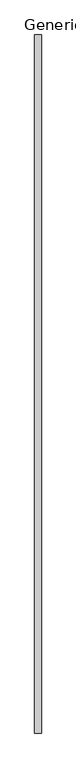
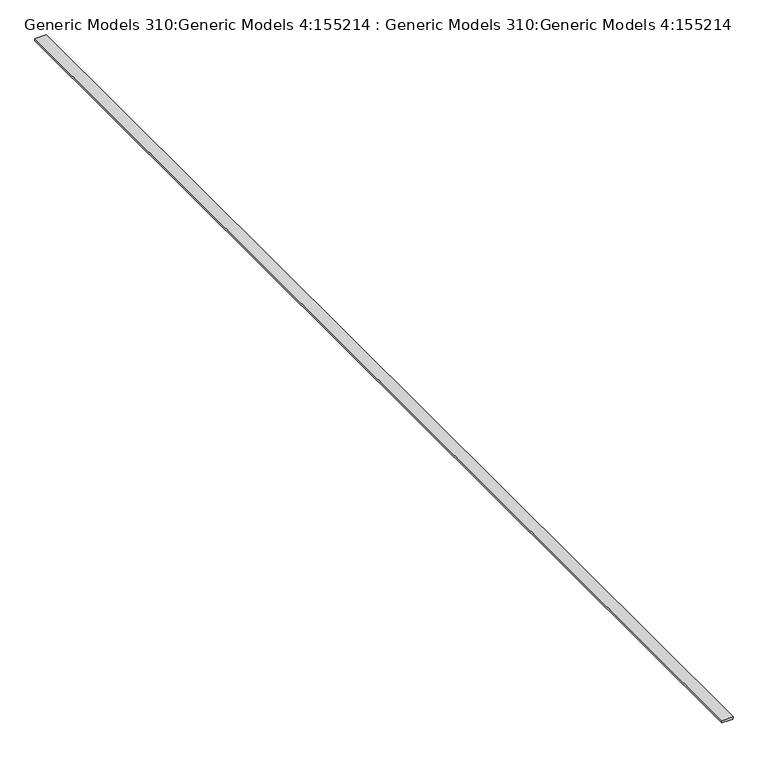
"""IFC4 building model written with IfcOpenShell, lengths in millimetres: proxy geometry, Generic Models 310:Generic Models 4:155214 : Generic Models 310:Generic Models 4:155214."""

from ifc_helpers import new_model, si_unit, frame, origin, place, context, project, spatial, polyline, outline, extrude, source, transform, mapped, element, save


def generic_models_310_generic_models_4_155214_generic_models_1d07e6d7(model_context):
    return source(origin(), model_context, "Body", "SweptSolid", [
        extrude(outline(polyline([(3057.525, 8521.578213), (3063.128839, 8521.578213), (3063.128839, 8437.0739977), (3044.825, 8437.0739977), (3044.825, 8497.8650291), (3046.095, 8497.8650291), (3046.095, 8520.308213), (3057.525, 8520.308213), (3057.525, 8521.578213)])), frame((0.0, -6674.7974793, 0.0), z_axis=(0.0, 1.0, 0.0), x_axis=(0.0, 0.0, 1.0)), (0.0, 0.0, 1.0), 8940.8),
    ])


if __name__ == "__main__":
    model = new_model("IFC4")
    model_context = context("Model", 3, world=origin())
    ifc_project = project(units=[si_unit("LENGTHUNIT", "METRE", prefix="MILLI")], contexts=[model_context])
    site = spatial("IfcSite", under=ifc_project)
    building = spatial("IfcBuilding", under=site)
    placement = place(None, origin())
    generic_models_310_generic_models_4_155214_generic_models_shape = generic_models_310_generic_models_4_155214_generic_models_1d07e6d7(model_context)
    element("IfcBuildingElementProxy", 1, Name="Generic Models 310:Generic Models 4:155214 : Generic Models 310:Generic Models 4:155214", ObjectType="Generic Models 310:Generic Models 4:155214 : Generic Models 310:Generic Models 4:155214", at=placement, inside=building, context=model_context, shape_type="MappedRepresentation", body=[
        mapped(generic_models_310_generic_models_4_155214_generic_models_shape, transform((0.0, 0.0, 0.0), x_axis=(1.0, 0.0, 0.0), y_axis=(0.0, 1.0, 0.0), z_axis=(0.0, 0.0, 1.0))),
    ])
    save(model, "model.ifc")

# Revit data of these elements
# Type "Generic Models 310:Generic Models 4:155214 : Generic Models 310:Generic Models 4:155214"
#   NameOverride = "Generic Models 310:Generic Models 4:155214"
#   ObjectTypeOverride = "Generic Models 310:Generic Models 4"
#   Reference = "Generic Models 4"
#   Category = "Generic Models"
#   Tag = "155214"
# Element 1 (IfcBuildingElementProxy, "Generic Models 310:Generic Models 4:155214 : Generic Models 310:Generic Models 4:155214")
#   Materials on its faces: "_7/8\" SMOOTH TROWEL EXTERIOR STUCCO (COLOR PER OWNER) 770"
# Materials
#   "_7/8\" SMOOTH TROWEL EXTERIOR STUCCO (COLOR PER OWNER) 770": class "Unassigned", colour RGB 233 233 233, transparency 0
